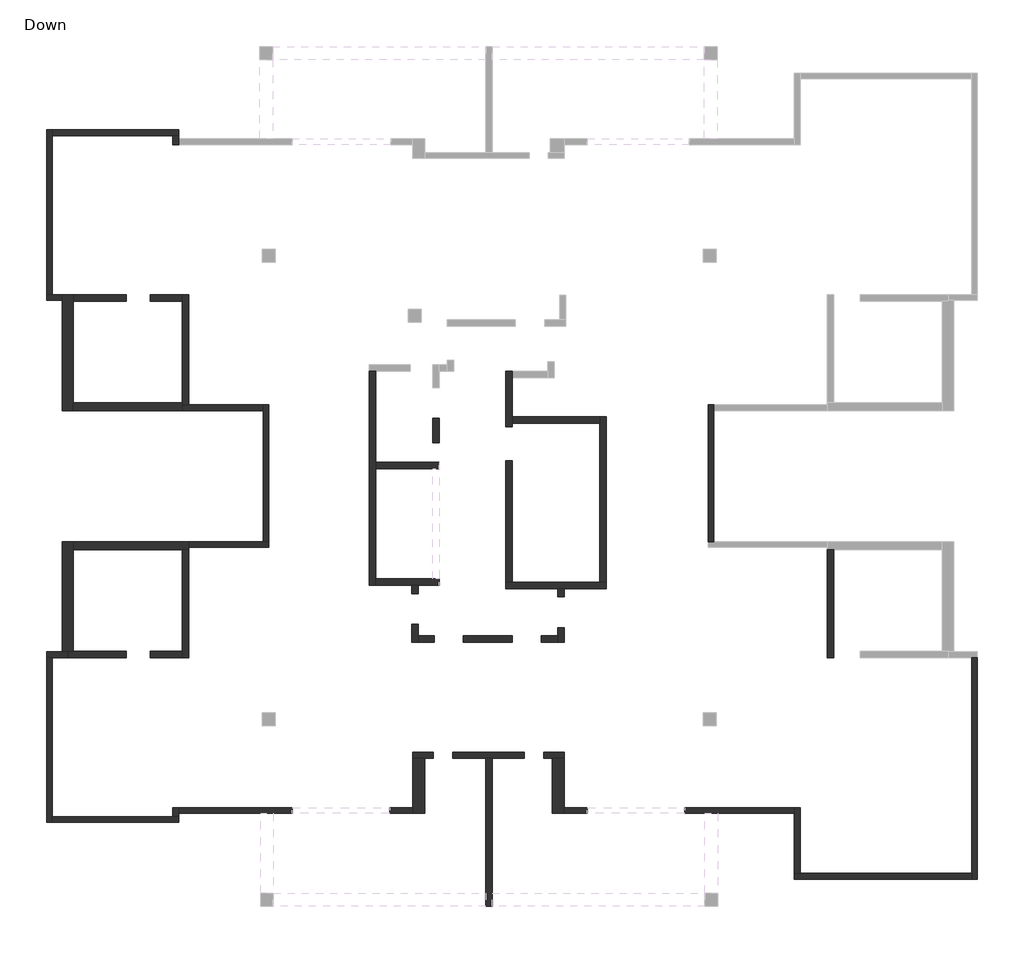
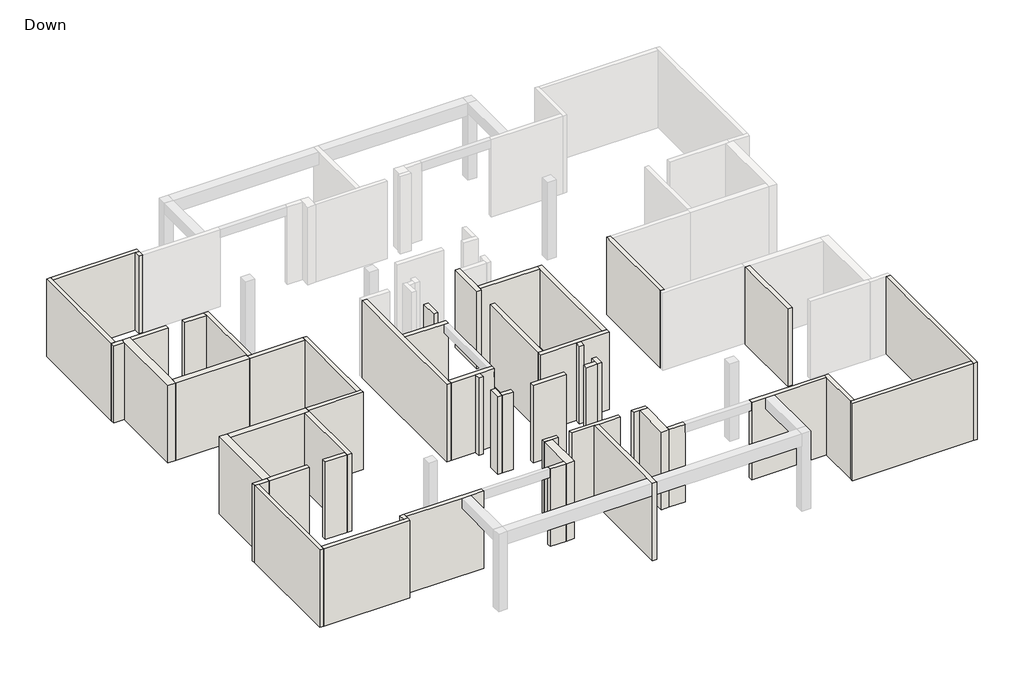
# One storey, part 1 of 2: 52 walls.
# Revit data of these elements (continued)
# Element 23 (IfcWall, "20") (continued)
#   SOFiSTiK_AMG_Scheduled = yes
#   SOFiSTiK_AMG_Adjusted = yes
#   Phase Created = New Construction
#   Base Constraint = Down
#   Top Constraint = Typical Floor
#   Materials on its faces: "Concrete"
# Element 24 (IfcWall, "20")
#   Comments = ""
#   Mark = "W41"
#   SOFiSTiK_EdgeZones = "W43"
#   SOFiSTiK_AMG_Comments = ""
#   Top Offset = 0 cm
#   Base Offset = 0 cm
#   wall height = 370 cm
#   SOFiSTiK_AMG_Scheduled = yes
#   SOFiSTiK_AMG_Adjusted = yes
#   Phase Created = New Construction
#   Base Constraint = Down
#   Top Constraint = Typical Floor
#   Materials on its faces: "Concrete"
# Element 25 (IfcWall, "20")
#   Comments = ""
#   Mark = "W42"
#   SOFiSTiK_EdgeZones = "W44"
#   SOFiSTiK_AMG_Comments = ""
#   Top Offset = 0 cm
#   Base Offset = 0 cm
#   wall height = 370 cm
#   SOFiSTiK_AMG_Scheduled = yes
#   SOFiSTiK_AMG_Adjusted = yes
#   Phase Created = New Construction
#   Base Constraint = Down
#   Top Constraint = Typical Floor
#   Materials on its faces: "Concrete"
# Element 26 (IfcWall, "20")
#   Comments = ""
#   Mark = "W43"
#   SOFiSTiK_EdgeZones = "W45"
#   SOFiSTiK_AMG_Comments = ""
#   Top Offset = 0 cm
#   Base Offset = 0 cm
#   wall height = 370 cm
#   SOFiSTiK_AMG_Scheduled = yes
#   SOFiSTiK_AMG_Adjusted = yes
#   Phase Created = New Construction
#   Base Constraint = Down
#   Top Constraint = Typical Floor
#   Materials on its faces: "Concrete"
# Element 27 (IfcWall, "20")
#   Comments = ""
#   Mark = "W45"
#   SOFiSTiK_EdgeZones = "W47"
#   SOFiSTiK_AMG_Comments = ""
#   Top Offset = 0 cm
#   Base Offset = 0 cm
#   wall height = 370 cm
#   SOFiSTiK_AMG_Scheduled = yes
#   SOFiSTiK_AMG_Adjusted = yes
#   Phase Created = New Construction
#   Base Constraint = Down
#   Top Constraint = Typical Floor
#   Materials on its faces: "Concrete"
# Element 28 (IfcWall, "20")
#   Comments = ""
#   Mark = "W46"
#   SOFiSTiK_EdgeZones = "W48"
#   SOFiSTiK_AMG_Comments = ""
#   Top Offset = 0 cm
#   Base Offset = 0 cm
#   wall height = 370 cm
#   SOFiSTiK_AMG_Scheduled = yes
#   SOFiSTiK_AMG_Adjusted = yes
#   Phase Created = New Construction
#   Base Constraint = Down
#   Top Constraint = Typical Floor
#   Materials on its faces: "Concrete"
# Element 29 (IfcWall, "20")
#   Comments = ""
#   Mark = "W47"
#   SOFiSTiK_EdgeZones = "W49"
#   SOFiSTiK_AMG_Comments = ""
#   Top Offset = 0 cm
#   Base Offset = 0 cm
#   wall height = 370 cm
#   SOFiSTiK_AMG_Scheduled = yes
#   SOFiSTiK_AMG_Adjusted = yes
#   Phase Created = New Construction
#   Base Constraint = Down
#   Top Constraint = Typical Floor
#   Materials on its faces: "Concrete"
# Element 30 (IfcWall, "20")
#   Comments = ""
#   Mark = "W48"
#   SOFiSTiK_EdgeZones = "W50"
#   SOFiSTiK_AMG_Comments = ""
#   Top Offset = 0 cm
#   Base Offset = 0 cm
#   wall height = 370 cm
#   SOFiSTiK_AMG_Scheduled = yes
#   SOFiSTiK_AMG_Adjusted = yes
#   Phase Created = New Construction
#   Base Constraint = Down
#   Top Constraint = Typical Floor
#   Materials on its faces: "Concrete"
# Element 31 (IfcWall, "20")
#   Comments = ""
#   Mark = "W52"
#   SOFiSTiK_EdgeZones = "W54"
#   SOFiSTiK_AMG_Comments = ""
#   Top Offset = 0 cm
#   Base Offset = 0 cm
#   wall height = 370 cm
#   SOFiSTiK_AMG_Scheduled = yes
#   SOFiSTiK_AMG_Adjusted = yes
#   Phase Created = New Construction
#   Base Constraint = Down
#   Top Constraint = Typical Floor
#   Materials on its faces: "Concrete"
# Element 32 (IfcWall, "20")
#   Comments = ""
#   Mark = "W53"
#   SOFiSTiK_EdgeZones = "W55"
#   SOFiSTiK_AMG_Comments = ""
#   Top Offset = 0 cm
#   Base Offset = 0 cm
#   wall height = 370 cm
#   SOFiSTiK_AMG_Scheduled = yes
#   SOFiSTiK_AMG_Adjusted = yes
#   Phase Created = New Construction
#   Base Constraint = Down
#   Top Constraint = Typical Floor
#   Materials on its faces: "Concrete"
# Element 33 (IfcWall, "20")
#   Comments = ""
#   Mark = "W54"
#   SOFiSTiK_EdgeZones = "W56"
#   SOFiSTiK_AMG_Comments = ""
#   Top Offset = 0 cm
#   Base Offset = 0 cm
#   wall height = 370 cm
#   SOFiSTiK_AMG_Scheduled = yes
#   SOFiSTiK_AMG_Adjusted = yes
#   Phase Created = New Construction
#   Base Constraint = Down
#   Top Constraint = Typical Floor
#   Materials on its faces: "Concrete"
# Element 34 (IfcWall, "20")
#   Comments = ""
#   Mark = "W55"
#   SOFiSTiK_EdgeZones = "W57"
#   SOFiSTiK_AMG_Comments = ""
#   Top Offset = 0 cm
#   Base Offset = 0 cm
#   wall height = 370 cm
#   SOFiSTiK_AMG_Scheduled = yes
#   SOFiSTiK_AMG_Adjusted = yes
#   Phase Created = New Construction
#   Base Constraint = Down
#   Top Constraint = Typical Floor
#   Materials on its faces: "Concrete"
# Element 35 (IfcWall, "20")
#   Comments = ""
#   Mark = "W56"
#   SOFiSTiK_EdgeZones = "W58"
#   SOFiSTiK_AMG_Comments = ""
#   Top Offset = 0 cm
#   Base Offset = 0 cm
#   wall height = 370 cm
#   SOFiSTiK_AMG_Scheduled = yes
#   SOFiSTiK_AMG_Adjusted = yes
#   Phase Created = New Construction
#   Base Constraint = Down
#   Top Constraint = Typical Floor
#   Materials on its faces: "Concrete"
# Element 36 (IfcWall, "20")
#   Comments = ""
#   Mark = "W57"
#   SOFiSTiK_EdgeZones = "W59"
#   SOFiSTiK_AMG_Comments = ""
#   Top Offset = 0 cm
#   Base Offset = 0 cm
#   wall height = 370 cm
#   SOFiSTiK_AMG_Scheduled = yes
#   SOFiSTiK_AMG_Adjusted = yes
#   Phase Created = New Construction
#   Base Constraint = Down
#   Top Constraint = Typical Floor
#   Materials on its faces: "Concrete"
# Element 37 (IfcWall, "20")
#   Comments = ""
#   Mark = "W58"
#   SOFiSTiK_EdgeZones = "W60"
#   SOFiSTiK_AMG_Comments = ""
#   Top Offset = 0 cm
#   Base Offset = 0 cm
#   wall height = 370 cm
#   SOFiSTiK_AMG_Scheduled = yes
#   SOFiSTiK_AMG_Adjusted = yes
#   Phase Created = New Construction
#   Base Constraint = Down
#   Top Constraint = Typical Floor
#   Materials on its faces: "Concrete"
# Element 38 (IfcWall, "20")
#   Comments = ""
#   Mark = "W59"
#   SOFiSTiK_EdgeZones = "W61"
#   SOFiSTiK_AMG_Comments = ""
#   Top Offset = 0 cm
#   Base Offset = 0 cm
#   wall height = 370 cm
#   SOFiSTiK_AMG_Scheduled = yes
#   SOFiSTiK_AMG_Adjusted = yes
#   Phase Created = New Construction
#   Base Constraint = Down
#   Top Constraint = Typical Floor
#   Materials on its faces: "Concrete"
# Element 39 (IfcWall, "20")
#   Comments = ""
#   Mark = "W60"
#   SOFiSTiK_EdgeZones = "W62"
#   SOFiSTiK_AMG_Comments = ""
#   Top Offset = 0 cm
#   Base Offset = 0 cm
#   wall height = 370 cm
#   SOFiSTiK_AMG_Scheduled = yes
#   SOFiSTiK_AMG_Adjusted = yes
#   Phase Created = New Construction
#   Base Constraint = Down
#   Top Constraint = Typical Floor
#   Materials on its faces: "Concrete"
# Element 40 (IfcWall, "20")
#   Comments = ""
#   Mark = "W61"
#   SOFiSTiK_EdgeZones = "W63"
#   SOFiSTiK_AMG_Comments = ""
#   Top Offset = 0 cm
#   Base Offset = 0 cm
#   wall height = 370 cm
#   SOFiSTiK_AMG_Scheduled = yes
#   SOFiSTiK_AMG_Adjusted = yes
#   Phase Created = New Construction
#   Base Constraint = Down
#   Top Constraint = Typical Floor
#   Materials on its faces: "Concrete"
# Element 41 (IfcWall, "20")
#   Comments = ""
#   Mark = "W62"
#   SOFiSTiK_EdgeZones = "W64"
#   SOFiSTiK_AMG_Comments = ""
#   Top Offset = 0 cm
#   Base Offset = 0 cm
#   wall height = 370 cm
#   SOFiSTiK_AMG_Scheduled = yes
#   SOFiSTiK_AMG_Adjusted = yes
#   Phase Created = New Construction
#   Base Constraint = Down
#   Top Constraint = Typical Floor
#   Materials on its faces: "Concrete"
# Element 42 (IfcWall, "20")
#   Comments = ""
#   Mark = "W63"
#   SOFiSTiK_EdgeZones = "W65"
#   SOFiSTiK_AMG_Comments = ""
#   Top Offset = 0 cm
#   Base Offset = 0 cm
#   wall height = 370 cm
#   SOFiSTiK_AMG_Scheduled = yes
#   SOFiSTiK_AMG_Adjusted = yes
#   Phase Created = New Construction
#   Base Constraint = Down
#   Top Constraint = Typical Floor
#   Materials on its faces: "Concrete"
# Element 43 (IfcWall, "20")
#   Comments = ""
#   Mark = "W71"
#   SOFiSTiK_EdgeZones = "W73"
#   SOFiSTiK_AMG_Comments = ""
#   Top Offset = 0 cm
#   Base Offset = 0 cm
#   wall height = 370 cm
#   SOFiSTiK_AMG_Scheduled = yes
#   SOFiSTiK_AMG_Adjusted = yes
#   Phase Created = New Construction
#   Base Constraint = Down
#   Top Constraint = Typical Floor
#   Materials on its faces: "Concrete"
# Element 44 (IfcWall, "20")
#   Comments = ""
#   Mark = "W73"
#   SOFiSTiK_EdgeZones = "W75"
#   SOFiSTiK_AMG_Comments = ""
#   Top Offset = 0 cm
#   Base Offset = 0 cm
#   wall height = 370 cm
#   SOFiSTiK_AMG_Scheduled = yes
#   SOFiSTiK_AMG_Adjusted = yes
#   Phase Created = New Construction
#   Base Constraint = Down
#   Top Constraint = Typical Floor
#   Materials on its faces: "Concrete"
# Element 45 (IfcWall, "20")
#   Comments = ""
#   Mark = "W74"
#   SOFiSTiK_EdgeZones = "W76"
#   SOFiSTiK_AMG_Comments = ""
#   Top Offset = 0 cm
#   Base Offset = 0 cm
#   wall height = 370 cm
#   SOFiSTiK_AMG_Scheduled = yes
#   SOFiSTiK_AMG_Adjusted = yes
#   Phase Created = New Construction
#   Base Constraint = Down
#   Top Constraint = Typical Floor
#   Materials on its faces: "Concrete"
# Element 46 (IfcWall, "20")
#   Comments = ""
#   Mark = "W75"
#   SOFiSTiK_EdgeZones = "W77"
#   SOFiSTiK_AMG_Comments = ""
#   Top Offset = 0 cm
#   Base Offset = 0 cm
#   wall height = 370 cm
#   SOFiSTiK_AMG_Scheduled = yes
#   SOFiSTiK_AMG_Adjusted = yes
#   Phase Created = New Construction
#   Base Constraint = Down
#   Top Constraint = Typical Floor
#   Materials on its faces: "Concrete"
# Element 47 (IfcWall, "25")
#   Comments = ""
#   Mark = "W80"
#   SOFiSTiK_EdgeZones = "W82"
#   SOFiSTiK_AMG_Comments = ""
#   Top Offset = 0 cm
#   Base Offset = 0 cm
#   wall height = 370 cm
#   SOFiSTiK_AMG_Scheduled = yes
#   SOFiSTiK_AMG_Adjusted = yes
#   Phase Created = New Construction
#   Base Constraint = Down
#   Top Constraint = Typical Floor
#   Materials on its faces: "Concrete"
# Element 48 (IfcWall, "25")
#   Comments = ""
#   Mark = "W82"
#   SOFiSTiK_EdgeZones = "W84"
#   SOFiSTiK_AMG_Comments = ""
#   Top Offset = 0 cm
#   Base Offset = 0 cm
#   wall height = 370 cm
#   SOFiSTiK_AMG_Scheduled = yes
#   SOFiSTiK_AMG_Adjusted = yes
#   Phase Created = New Construction
#   Base Constraint = Down
#   Top Constraint = Typical Floor
#   Materials on its faces: "Concrete"
# Element 49 (IfcWall, "35")
#   Comments = ""
#   Mark = "W76"
#   SOFiSTiK_EdgeZones = "W78"
#   SOFiSTiK_AMG_Comments = ""
#   Top Offset = 0 cm
#   Base Offset = 0 cm
#   wall height = 370 cm
#   SOFiSTiK_AMG_Scheduled = yes
#   SOFiSTiK_AMG_Adjusted = yes
#   Phase Created = New Construction
#   Base Constraint = Down
#   Top Constraint = Typical Floor
#   Materials on its faces: "Concrete"
# Element 50 (IfcWall, "35")
#   Comments = ""
#   Mark = "W78"
#   SOFiSTiK_EdgeZones = "W80"
#   SOFiSTiK_AMG_Comments = ""
#   Top Offset = 0 cm
#   Base Offset = 0 cm
#   wall height = 370 cm
#   SOFiSTiK_AMG_Scheduled = yes
#   SOFiSTiK_AMG_Adjusted = yes
#   Phase Created = New Construction
#   Base Constraint = Down
#   Top Constraint = Typical Floor
#   Materials on its faces: "Concrete"
# Element 51 (IfcWall, "36")
#   Comments = ""
#   Mark = "W37"
#   SOFiSTiK_EdgeZones = "W39"
#   SOFiSTiK_AMG_Comments = ""
#   Top Offset = 0 cm
#   Base Offset = 0 cm
#   wall height = 370 cm
#   SOFiSTiK_AMG_Scheduled = yes
#   SOFiSTiK_AMG_Adjusted = yes
#   Phase Created = New Construction
#   Base Constraint = Down
#   Top Constraint = Typical Floor
#   Materials on its faces: "Concrete"
# Element 52 (IfcWall, "36")
#   Comments = ""
#   Mark = "W38"
#   SOFiSTiK_EdgeZones = "W40"
#   SOFiSTiK_AMG_Comments = ""
#   Top Offset = 0 cm
#   Base Offset = 0 cm
#   wall height = 370 cm
#   SOFiSTiK_AMG_Scheduled = yes
#   SOFiSTiK_AMG_Adjusted = yes
#   Phase Created = New Construction
#   Base Constraint = Down
#   Top Constraint = Typical Floor
#   Materials on its faces: "Concrete"
# Materials
#   "Concrete": class "Concrete", colour RGB 192 192 192, transparency 0, Keynote = "01000", Description = "Cast-in-place concrete", Cost = 0
